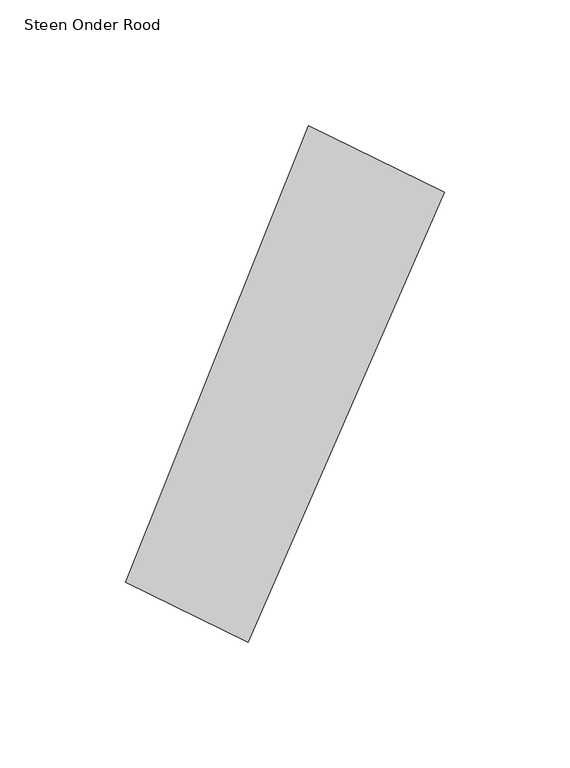
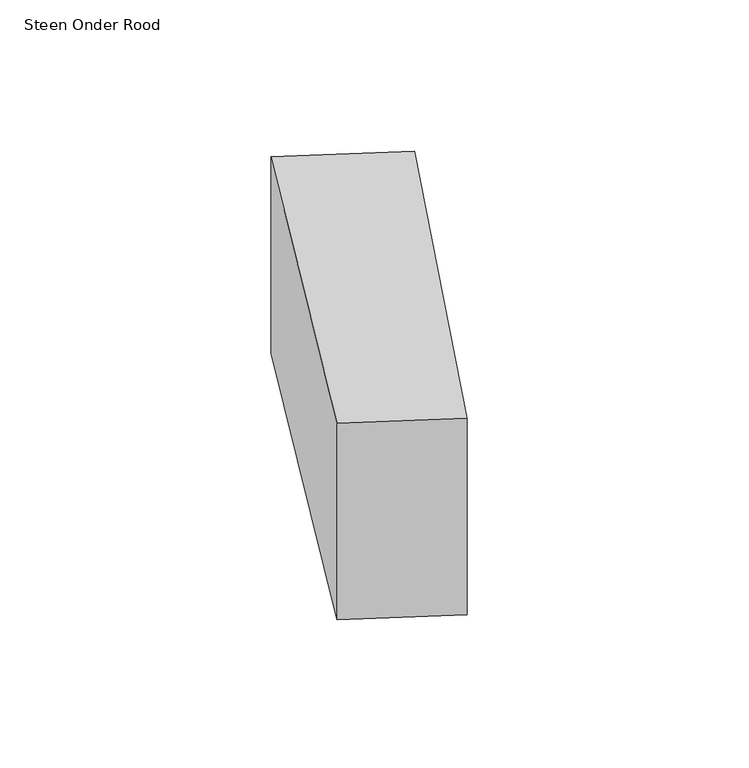
"""IFC4 building model written with IfcOpenShell, lengths in millimetres: proxy geometry, 00_GMA_steen_versie_4 : Steen Onder Rood."""

from ifc_helpers import new_model, si_unit, origin, origin_with_axes, place, context, project, spatial, polyline, outline, extrude, source, transform, mapped, element, save


def steen_onder_rood_0ae051be(model_context):
    return source(origin(), model_context, "Body", "SweptSolid", [
        extrude(outline(polyline([(139.0405462, 157.9754253), (61.0849714, -20.9746876), (12.2942705, 2.8746928), (85.1314098, 184.3348558), (139.0405462, 157.9754253)])), origin_with_axes(), (0.0, 0.0, 1.0), 100.0),
    ])


if __name__ == "__main__":
    model = new_model("IFC4")
    model_context = context("Model", 3, world=origin())
    ifc_project = project(units=[si_unit("LENGTHUNIT", "METRE", prefix="MILLI")], contexts=[model_context])
    site = spatial("IfcSite", under=ifc_project)
    building = spatial("IfcBuilding", under=site)
    placement = place(None, origin())
    steen_onder_rood_shape = steen_onder_rood_0ae051be(model_context)
    element("IfcBuildingElementProxy", 1, Name="00_GMA_steen_versie_4 : Steen Onder Rood", ObjectType="00_GMA_steen_versie_4 : Steen Onder Rood", at=placement, inside=building, context=model_context, shape_type="MappedRepresentation", body=[
        mapped(steen_onder_rood_shape, transform((0.0, 0.0, 0.0), x_axis=(1.0, 0.0, 0.0), y_axis=(0.0, 1.0, 0.0), z_axis=(0.0, 0.0, 1.0))),
    ])
    save(model, "model.ifc")

# Revit data of these elements
# Type "00_GMA_steen_versie_4 : Steen Onder Rood"
#   StootVoegHalfBoven [instance default] = 5 mm
#   StootVoegHalf [instance default] = 5 mm
#   StootVoegBreedteOnder = 10 mm
#   StootVoegBreedteBoven = 10 mm
#   Steendikte = 100 mm
#   LintVoegOnderHalf = 0 mm
#   LintVoegOnder = 0 mm
#   LintVoegBovenHalf = 5 mm
#   LintVoegBoven = 10 mm
#   materiaal = 21_steen_rood
#   MateriaalVoeg = none
#   Default Elevation = 0
# Element 1 (IfcBuildingElementProxy, "00_GMA_steen_versie_4 : Steen Onder Rood")
#   Materials on its faces: "21_steen_rood"
# Materials
#   "21_steen_rood": class "Unassigned", colour RGB 213 111 43, transparency 0, Cost = 0
